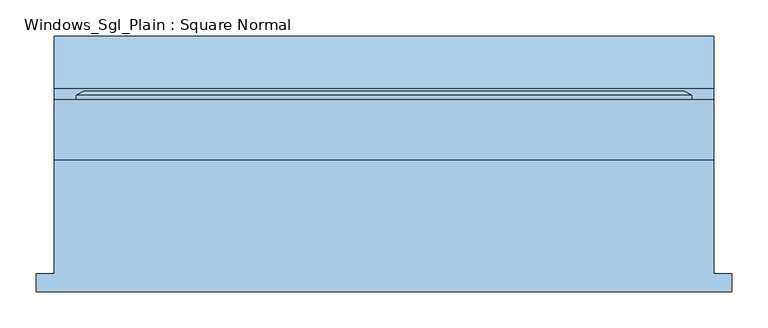
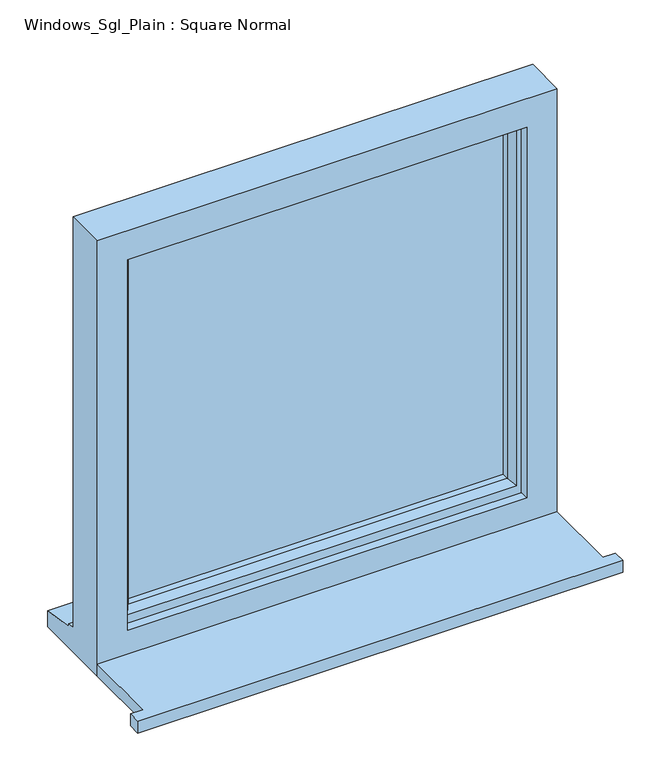
"""IFC4 building model written with IfcOpenShell, lengths in millimetres: window geometry, Windows_Sgl_Plain : Square Normal."""

from ifc_helpers import new_model, si_unit, frame, origin, place, context, project, spatial, polyline, outline, extrude, faceted_brep, source, transform, mapped, element, save


def windows_sgl_plain_square_normal_b9caa461(model_context):
    return source(origin(), model_context, "Body", "SolidModel", [
        extrude(outline(polyline([(-480.0, -161.5434322), (-480.0, -136.5434322), (-455.0, -136.5434322), (-455.0, 20.4565678), (455.0, 20.4565678), (455.0, -136.5434322), (480.0, -136.5434322), (480.0, -161.5434322), (-480.0, -161.5434322)])), frame((0.0, 0.0, 1200.0), z_axis=(0.0, 0.0, 1.0), x_axis=(1.0, 0.0, 0.0)), (0.0, 0.0, 1.0), 25.0),
        faceted_brep([(-455.0, 20.4565678, 1200.0), (455.0, 20.4565678, 1200.0), (455.0, 20.4565678, 2110.0), (-455.0, 20.4565678, 2110.0), (-395.0, 20.4565678, 2050.0), (395.0, 20.4565678, 2050.0), (395.0, 20.4565678, 1275.0), (-395.0, 20.4565678, 1275.0), (-455.0, 103.4565678, 2110.0), (-455.0, 103.4565678, 1251.0), (-455.0, 118.4565678, 1249.68767), (-455.0, 118.4565678, 1244.7449676), (-455.0, 190.9565678, 1233.8088847), (-455.0, 190.9565678, 1200.0), (455.0, 103.4565678, 2110.0), (455.0, 103.4565678, 1251.0), (-415.0, 103.4565678, 2070.0), (-415.0, 103.4565678, 1263.0), (415.0, 103.4565678, 1263.0), (415.0, 103.4565678, 2070.0), (-415.0, 38.4565678, 2070.0), (-415.0, 38.4565678, 1263.0), (415.0, 38.4565678, 2070.0), (415.0, 38.4565678, 1263.0), (-395.0, 38.4565678, 2050.0), (-395.0, 38.4565678, 1275.0), (395.0, 38.4565678, 1275.0), (395.0, 38.4565678, 2050.0), (455.0, 190.9565678, 1200.0), (455.0, 190.9565678, 1233.8088847), (455.0, 118.4565678, 1244.7449676), (455.0, 118.4565678, 1249.68767)], [[[0, 1, 2, 3], [4, 5, 6, 7]], [[0, 3, 8, 9, 10, 11, 12, 13]], [[9, 8, 14, 15], [16, 17, 18, 19]], [[17, 16, 20, 21]], [[20, 22, 23, 21], [24, 25, 26, 27]], [[24, 4, 7, 25]], [[3, 2, 14, 8]], [[16, 19, 22, 20]], [[5, 4, 24, 27]], [[15, 14, 2, 1, 28, 29, 30, 31]], [[19, 18, 23, 22]], [[5, 27, 26, 6]], [[28, 1, 0, 13]], [[29, 28, 13, 12]], [[30, 29, 12, 11]], [[31, 30, 11, 10]], [[15, 31, 10, 9]], [[21, 23, 18, 17]], [[7, 6, 26, 25]]]),
        extrude(outline(polyline([(385.0, 67.4565678), (-385.0, 67.4565678), (-385.0, 91.4565678), (385.0, 91.4565678), (385.0, 67.4565678)])), frame((0.0, 0.0, 1293.0), z_axis=(0.0, 0.0, 1.0), x_axis=(1.0, 0.0, 0.0)), (0.0, 0.0, 1.0), 747.0),
        faceted_brep([(-425.0, 103.4565678, 2080.0), (-425.0, 109.2300705, 2080.0), (-425.0, 109.2300705, 1253.0), (-425.0, 103.4565678, 1253.0), (-415.0, 38.4565678, 2070.0), (-415.0, 103.4565678, 2070.0), (-415.0, 103.4565678, 1263.0), (-415.0, 38.4565678, 1263.0), (-375.0, 52.9494677, 2030.0), (-385.1480377, 38.4565678, 2040.1480377), (-385.1480377, 38.4565678, 1292.8519623), (-375.0, 52.9494677, 1303.0), (-375.0, 67.4565678, 2030.0), (-375.0, 67.4565678, 1303.0), (-385.0, 91.4565678, 2040.0), (-385.0, 67.4565678, 2040.0), (-385.0, 67.4565678, 1293.0), (-385.0, 91.4565678, 1293.0), (-375.0, 109.2300705, 2030.0), (-375.0, 91.4565678, 2030.0), (-375.0, 91.4565678, 1303.0), (-375.0, 109.2300705, 1303.0), (-392.4457548, 115.0035732, 2047.4457548), (-392.4457548, 115.0035732, 1285.5542452), (-414.2153903, 115.0035732, 2069.2153903), (-414.2153903, 115.0035732, 1263.7846097), (425.0, 109.2300705, 1253.0), (425.0, 103.4565678, 1253.0), (415.0, 103.4565678, 1263.0), (415.0, 38.4565678, 1263.0), (385.1480377, 38.4565678, 1292.8519623), (375.0, 52.9494677, 1303.0), (375.0, 67.4565678, 1303.0), (385.0, 67.4565678, 1293.0), (385.0, 91.4565678, 1293.0), (375.0, 91.4565678, 1303.0), (375.0, 109.2300705, 1303.0), (392.4457548, 115.0035732, 1285.5542452), (414.2153903, 115.0035732, 1263.7846097), (425.0, 109.2300705, 2080.0), (425.0, 103.4565678, 2080.0), (415.0, 103.4565678, 2070.0), (415.0, 38.4565678, 2070.0), (385.1480377, 38.4565678, 2040.1480377), (375.0, 52.9494677, 2030.0), (375.0, 67.4565678, 2030.0), (385.0, 67.4565678, 2040.0), (385.0, 91.4565678, 2040.0), (375.0, 91.4565678, 2030.0), (375.0, 109.2300705, 2030.0), (392.4457548, 115.0035732, 2047.4457548), (414.2153903, 115.0035732, 2069.2153903)], [[[0, 1, 2, 3]], [[4, 5, 6, 7]], [[8, 9, 10, 11]], [[12, 8, 11, 13]], [[14, 15, 16, 17]], [[18, 19, 20, 21]], [[22, 18, 21, 23]], [[1, 24, 25, 2]], [[3, 2, 26, 27]], [[7, 6, 28, 29]], [[11, 10, 30, 31]], [[13, 11, 31, 32]], [[17, 16, 33, 34]], [[21, 20, 35, 36]], [[23, 21, 36, 37]], [[2, 25, 38, 26]], [[27, 26, 39, 40]], [[29, 28, 41, 42]], [[31, 30, 43, 44]], [[32, 31, 44, 45]], [[34, 33, 46, 47]], [[36, 35, 48, 49]], [[37, 36, 49, 50]], [[26, 38, 51, 39]], [[40, 39, 1, 0]], [[3, 27, 40, 0], [5, 41, 28, 6]], [[42, 41, 5, 4]], [[7, 29, 42, 4], [9, 43, 30, 10]], [[44, 43, 9, 8]], [[45, 44, 8, 12]], [[15, 46, 33, 16], [13, 32, 45, 12]], [[47, 46, 15, 14]], [[17, 34, 47, 14], [19, 48, 35, 20]], [[49, 48, 19, 18]], [[50, 49, 18, 22]], [[24, 51, 38, 25], [23, 37, 50, 22]], [[39, 51, 24, 1]]]),
    ])


if __name__ == "__main__":
    model = new_model("IFC4")
    model_context = context("Model", 3, world=origin())
    ifc_project = project(units=[si_unit("LENGTHUNIT", "METRE", prefix="MILLI")], contexts=[model_context])
    site = spatial("IfcSite", under=ifc_project)
    building = spatial("IfcBuilding", under=site)
    placement = place(None, origin())
    windows_sgl_plain_square_normal_shape = windows_sgl_plain_square_normal_b9caa461(model_context)
    element("IfcWindow", 1, ObjectType="Windows_Sgl_Plain : Square Normal", at=placement, inside=building, context=model_context, shape_type="MappedRepresentation", body=[
        mapped(windows_sgl_plain_square_normal_shape, transform((0.0, 0.0, 0.0), x_axis=(1.0, 0.0, 0.0), y_axis=(0.0, 1.0, 0.0), z_axis=(0.0, 0.0, 1.0))),
    ])
    save(model, "model.ifc")

# Revit data of these elements
# Project information
#   Project Issue Date = "Issue Date"
#   Project Status = "Project Status"
#   Client Name = "Owner"
#   Project Address = "Enter address here"
#   Project Name = "Project Name"
#   Project Number = "Project Number"
# Type "Windows_Sgl_Plain : Square Normal"
#   Type Mark = "44"
#   Operation = "SinglePanel"
#   Construction Type Id = "SGL"
#   Manufacturer = "Revit"
#   Keynote = "L10"
#   Analytic Construction = "Large single-glazed windows"
#   Wrap Layers (Ext) from Ext = 102.5 mm
#   Wrap Layers (Int) from Ext = 177.5 mm
#   Window Board Projection = 25 mm
#   Window Board Extension = 25 mm
#   Visual Light Transmittance = 0.9
#   Solar Heat Gain Coefficient = 0.86
#   Rough Width = 910 mm
#   Rough Height = 910 mm
#   Height = 910 mm
#   Width = 910 mm
#   Heat Transfer Coefficient (U) = 5.5617 W/(m²·K)
#   Glazing Thickness = 24 mm
#   FrameOffset - External = 50 mm
#   Frame Depth = 65 mm
#   Default Head Height = 2110 mm
#   Cill Depth = 87.5 mm
#   Cavity Closer Width = 50 mm
#   Cavity Closer Offset from Ext = 102.5 mm
#   Cavity Closer Depth = 85 mm
#   Vis - Cavity Closers = yes
#   Material Trim = Window Frame
#   Material Glass = Glass
#   Material Frame = Window Frame
#   Wall Closure = (empty or 0)
# Element 1 (IfcWindow, "Windows_Sgl_Plain : Square Normal")
#   Materials on its faces: "Window Frame", "Glass"
# Materials
#   "Window Frame": class "Miscellaneous", colour RGB 249 249 249, transparency 0, Keynote = "L10", Cost = 0
#   "Glass": class "Glass", colour RGB 0 128 192, transparency 0.9, Description = "Soda Lime Glass", Cost = 0
